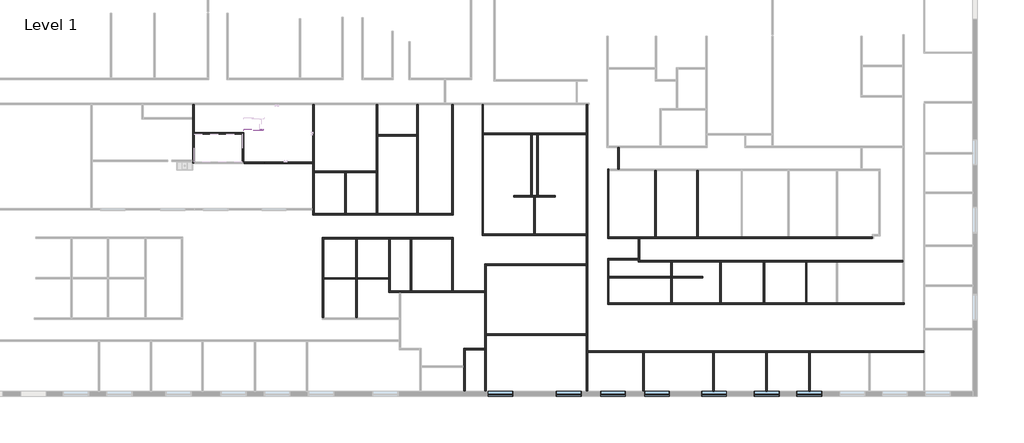
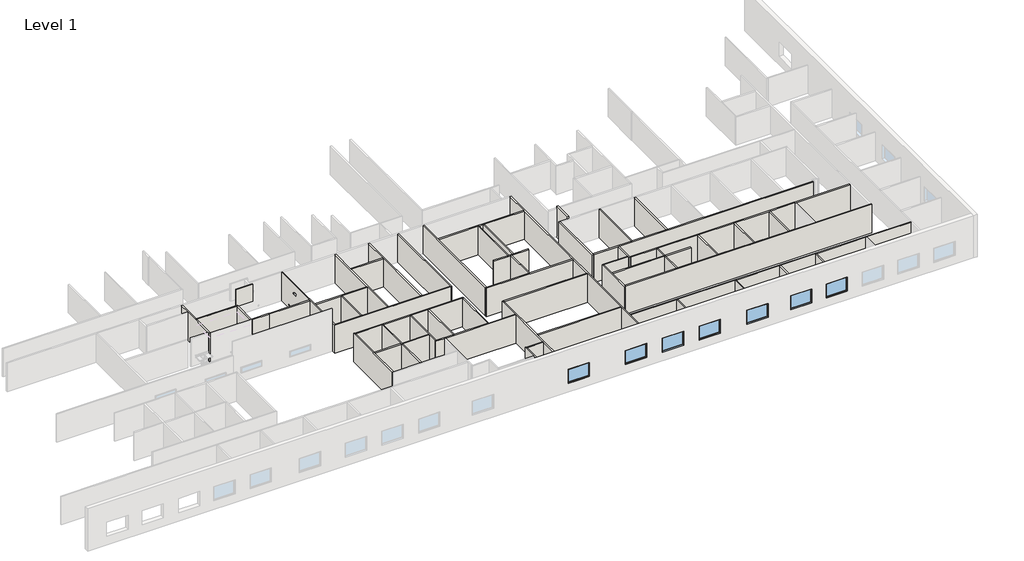
# One storey, part 2 of 4: 55 walls, 7 windows.
# Revit data of these elements (continued)
# Element 17 (IfcWall, "Interior - 4 7/8\" Partition (1-hr)")
#   built-in parameter 1001111 = 9' - 0"
#   Top Offset = 0' - 0"
#   Base Offset = 9' - 0"
#   Unconnected Height = 6' - 0"
#   wall height = 6' - 0"
#   Phase Created = 03 - Project Completion
#   Base Constraint = Level 1
#   Materials on its faces: "Default Wall", "Gypsum Wall Board"
# Elements 18, 19, 22, 30, 32, 34, 47 (IfcWall, "Interior - 4 7/8\" Partition (1-hr)")
#   Top Offset = 0' - 0"
#   Base Offset = 0' - 0"
#   Unconnected Height = 10' - 0"
#   wall height = 10' - 0"
#   Phase Created = 03 - Project Completion
#   Base Constraint = Level 1
#   Materials on its faces: "Gypsum Wall Board", "Default Wall"
# Element 55 (IfcWall, "Interior - 4 7/8\" Partition (1-hr)")
#   built-in parameter 1001111 = -0' - 1.98797"
#   Top Offset = 0' - 0"
#   Base Offset = -0' - 1.98797"
#   Unconnected Height = 10' - 11.88518"
#   wall height = 10' - 11.88518"
#   Phase Created = 03 - Project Completion
#   Base Constraint = Level 1
#   Materials on its faces: "Default Wall", "Gypsum Wall Board"
# Element 56 (IfcWindow, "Fixed : 86\" x 60\"")
#   Mark = "14"
#   Phase Created = 01 - Existing
#   Materials on its faces: "Sash", "Glass"
# Element 57 (IfcWindow, "Fixed : 86\" x 60\"")
#   Mark = "15"
#   Phase Created = 01 - Existing
#   Materials on its faces: "Sash", "Glass"
# Element 58 (IfcWindow, "Fixed : 86\" x 60\"")
#   Mark = "16"
#   Phase Created = 01 - Existing
#   Materials on its faces: "Sash", "Glass"
# Element 59 (IfcWindow, "Fixed : 86\" x 60\"")
#   Mark = "17"
#   Phase Created = 01 - Existing
#   Materials on its faces: "Sash", "Glass"
# Element 60 (IfcWindow, "Fixed : 86\" x 60\"")
#   Mark = "18"
#   Phase Created = 01 - Existing
#   Materials on its faces: "Sash", "Glass"
# Element 61 (IfcWindow, "Fixed : 86\" x 60\"")
#   Mark = "19"
#   Phase Created = 01 - Existing
#   Materials on its faces: "Sash", "Glass"
# Element 62 (IfcWindow, "Fixed : 86\" x 60\"")
#   Mark = "20"
#   Phase Created = 01 - Existing
#   Materials on its faces: "Sash", "Glass"
# Materials
#   "Gypsum Wall Board": class "Generic", colour RGB 127 127 127, transparency 0, Description = "Gypsum Wall Board", Cost = 0
#   "Metal Stud Layer": class "Metal", colour RGB 199 199 199, transparency 0, Description = "Light gauge steel framing, thermal air layer", Cost = 0
#   "Glass": class "Glass", colour RGB 0 128 192, transparency 0.75, Description = "Soda Lime Glass", Cost = 0
#   "Sash": class "Wood", colour RGB 224 178 126, transparency 0
#   "Default Wall": class "Miscellaneous", colour RGB 128 128 128, transparency 0
